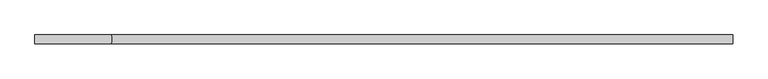
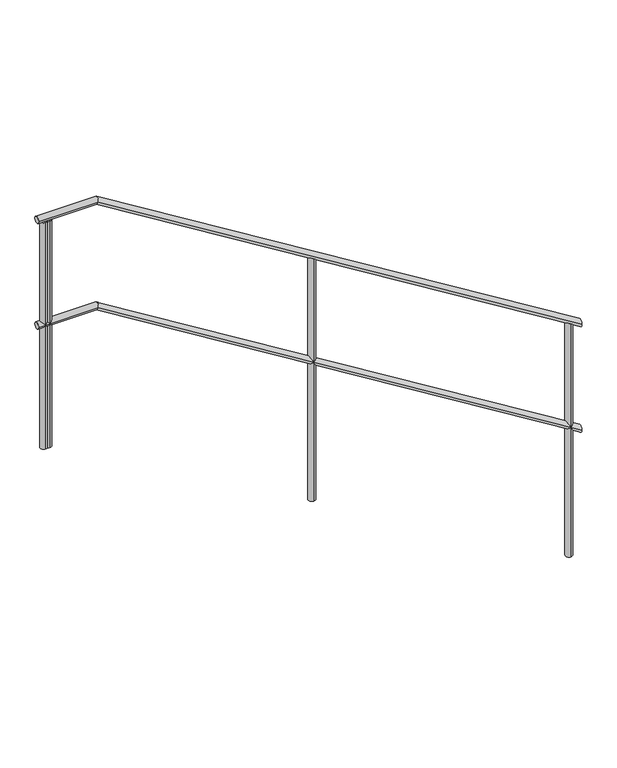
"""IFC4 building model written with IfcOpenShell, lengths in millimetres: railing geometry."""

from ifc_helpers import new_model, si_unit, point, frame, frame_2d, origin, place, context, project, spatial, circle_curve, ellipse_curve, trimmed, segment, composite_curve, outline, extrude, source, transform, mapped, element, save
from ifc_brep_helpers import plane_surface, cylinder_surface, advanced_brep


def railing_ed82b161(model_context):
    return source(origin(), model_context, "Body", "SolidModel", [
        advanced_brep(
        [(28470.0, -5867.9791411, -450.9609787), (28470.0, -5837.9791411, -450.9609787), (26305.7432145, -5867.9791411, 885.0), (26305.7432145, -5837.9791411, 885.0), (26040.0, -5867.9791411, 885.0), (26040.0, -5837.9791411, 885.0)],
        [
            (0, 1, ellipse_curve(frame((28470.0, -5852.9791411, -450.9609787), z_axis=(1.0, 0.0, 0.0), x_axis=(0.0, 0.0, -1.0)), 17.6276454, 15.0)),
            (1, 0, ellipse_curve(frame((28470.0, -5852.9791411, -450.9609787), z_axis=(1.0, 0.0, 0.0), x_axis=(0.0, 0.0, -1.0)), 17.6276454, 15.0)),
            (0, 2),
            (2, 3, ellipse_curve(frame((26305.7432145, -5852.9791411, 885.0), z_axis=(0.9620125025549406, 0.0, -0.27300539358770975), x_axis=(-0.27300539358770975, 0.0, -0.9620125025549406)), 15.5923129, 15.0)),
            (3, 1),
            (3, 2, ellipse_curve(frame((26305.7432145, -5852.9791411, 885.0), z_axis=(0.9620125025549406, 0.0, -0.27300539358770975), x_axis=(-0.27300539358770975, 0.0, -0.9620125025549406)), 15.5923129, 15.0)),
            (4, 5, circle_curve(frame((26040.0, -5852.9791411, 885.0), z_axis=(-1.0, 0.0, 0.0), x_axis=(0.0, 1.0, 0.0)), 15.0)),
            (5, 4, circle_curve(frame((26040.0, -5852.9791411, 885.0), z_axis=(-1.0, 0.0, 0.0), x_axis=(0.0, 1.0, 0.0)), 15.0)),
            (2, 4),
            (5, 3),
        ],
        [
            plane_surface(frame((28470.0, -5852.9791411, -433.3333333), z_axis=(1.0, 0.0, 0.0), x_axis=(0.0, -1.0, 0.0))),
            cylinder_surface(frame((28462.1209619, -5852.9791411, -446.097375), z_axis=(0.8509361101440394, 0.0, -0.5252692037926184), x_axis=(0.0, 1.0, 0.0)), 15.0),
            plane_surface(frame((26040.0, -5852.9791411, 900.0), z_axis=(-1.0, 0.0, 0.0), x_axis=(0.0, -1.0, 0.0))),
            cylinder_surface(frame((26310.0, -5852.9791411, 885.0), z_axis=(1.0, 0.0, 0.0), x_axis=(0.0, 1.0, 0.0)), 15.0),
        ],
        [
            (0, [[1, 2]]),
            (1, [[-1, 3, 4, 5]]),
            (1, [[-2, -5, 6, -3]]),
            (2, [[7, 8]]),
            (3, [[-4, 9, -8, 10]]),
            (3, [[-6, -10, -7, -9]]),
        ],
    ),
        advanced_brep(
        [(28470.0, -5867.9791411, 49.0390213), (28470.0, -5837.9791411, 49.0390213), (26305.7432145, -5867.9791411, 1385.0), (26305.7432145, -5837.9791411, 1385.0), (26040.0, -5867.9791411, 1385.0), (26040.0, -5837.9791411, 1385.0)],
        [
            (0, 1, ellipse_curve(frame((28470.0, -5852.9791411, 49.0390213), z_axis=(1.0, 0.0, 0.0), x_axis=(0.0, 0.0, -1.0)), 17.6276454, 15.0)),
            (1, 0, ellipse_curve(frame((28470.0, -5852.9791411, 49.0390213), z_axis=(1.0, 0.0, 0.0), x_axis=(0.0, 0.0, -1.0)), 17.6276454, 15.0)),
            (0, 2),
            (2, 3, ellipse_curve(frame((26305.7432145, -5852.9791411, 1385.0), z_axis=(0.9620125025549406, 0.0, -0.27300539358770975), x_axis=(-0.27300539358770975, 0.0, -0.9620125025549406)), 15.5923129, 15.0)),
            (3, 1),
            (3, 2, ellipse_curve(frame((26305.7432145, -5852.9791411, 1385.0), z_axis=(0.9620125025549406, 0.0, -0.27300539358770975), x_axis=(-0.27300539358770975, 0.0, -0.9620125025549406)), 15.5923129, 15.0)),
            (4, 5, circle_curve(frame((26040.0, -5852.9791411, 1385.0), z_axis=(-1.0, 0.0, 0.0), x_axis=(0.0, 1.0, 0.0)), 15.0)),
            (5, 4, circle_curve(frame((26040.0, -5852.9791411, 1385.0), z_axis=(-1.0, 0.0, 0.0), x_axis=(0.0, 1.0, 0.0)), 15.0)),
            (2, 4),
            (5, 3),
        ],
        [
            plane_surface(frame((28470.0, -5852.9791411, 66.6666667), z_axis=(1.0, 0.0, 0.0), x_axis=(0.0, -1.0, 0.0))),
            cylinder_surface(frame((28462.1209619, -5852.9791411, 53.902625), z_axis=(0.8509361101440394, 0.0, -0.5252692037926184), x_axis=(0.0, 1.0, 0.0)), 15.0),
            plane_surface(frame((26040.0, -5852.9791411, 1400.0), z_axis=(-1.0, 0.0, 0.0), x_axis=(0.0, -1.0, 0.0))),
            cylinder_surface(frame((26310.0, -5852.9791411, 1385.0), z_axis=(1.0, 0.0, 0.0), x_axis=(0.0, 1.0, 0.0)), 15.0),
        ],
        [
            (0, [[1, 2]]),
            (1, [[-1, 3, 4, 5]]),
            (1, [[-2, -5, 6, -3]]),
            (2, [[7, 8]]),
            (3, [[-4, 9, -8, 10]]),
            (3, [[-6, -10, -7, -9]]),
        ],
    ),
        extrude(outline(composite_curve([segment(trimmed(circle_curve(frame_2d((26070.0, -5852.9791411)), 15.0), [point((26070.0, -5867.9791411))], [point((26070.0, -5837.9791411))], False, "CARTESIAN"), True, "CONTINUOUS"), segment(trimmed(circle_curve(frame_2d((26070.0, -5852.9791411)), 15.0), [point((26070.0, -5837.9791411))], [point((26070.0, -5867.9791411))], False, "CARTESIAN"), True, "CONTINUOUS")], self_intersect=False)), frame((0.0, 0.0, 300.0), z_axis=(0.0, 0.0, 1.0), x_axis=(1.0, 0.0, 0.0)), (0.0, 0.0, 1.0), 1070.0),
        advanced_brep(
        [(27270.0, -5837.9791411, 777.4074074), (27270.0, -5837.9791411, -366.6666667), (27270.0, -5867.9791411, -366.6666667), (27270.0, -5867.9791411, 777.4074074)],
        [
            (0, 1),
            (1, 2, circle_curve(frame((27270.0, -5852.9791411, -366.6666667), z_axis=(0.0, 0.0, 1.0), x_axis=(0.0, -1.0, 0.0)), 15.0)),
            (2, 3),
            (3, 0, ellipse_curve(frame((27270.0, -5852.9791411, 777.4074074), z_axis=(-0.5252692037926167, 0.0, -0.8509361101440406), x_axis=(-0.8509361101440406, 0.0, 0.5252692037926162)), 17.6276454, 15.0)),
            (0, 3, ellipse_curve(frame((27270.0, -5852.9791411, 777.4074074), z_axis=(-0.5252692037926167, 0.0, -0.8509361101440406), x_axis=(-0.8509361101440406, 0.0, 0.5252692037926162)), 17.6276454, 15.0)),
            (2, 1, circle_curve(frame((27270.0, -5852.9791411, -366.6666667), z_axis=(0.0, 0.0, 1.0), x_axis=(0.0, -1.0, 0.0)), 15.0)),
        ],
        [
            cylinder_surface(frame((27270.0, -5852.9791411, -466.6666667), z_axis=(0.0, 0.0, 1.0), x_axis=(0.0, -1.0, 0.0)), 15.0),
            plane_surface(frame((27245.0, -5877.9791411, 792.8395062), z_axis=(0.5252692037926167, 0.0, 0.8509361101440406), x_axis=(0.0, 1.0, 0.0))),
            plane_surface(frame((27295.0, -5877.9791411, -366.6666667), z_axis=(0.0, 0.0, -1.0), x_axis=(0.0, 1.0, 0.0))),
        ],
        [
            (0, [[1, 2, 3, 4]]),
            (0, [[-1, 5, -3, 6]]),
            (1, [[-4, -5]]),
            (2, [[-2, -6]]),
        ],
    ),
        extrude(outline(composite_curve([segment(trimmed(circle_curve(frame_2d((26090.0, -5852.9791411)), 15.0), [point((26090.0, -5867.9791411))], [point((26090.0, -5837.9791411))], False, "CARTESIAN"), True, "CONTINUOUS"), segment(trimmed(circle_curve(frame_2d((26090.0, -5852.9791411)), 15.0), [point((26090.0, -5837.9791411))], [point((26090.0, -5867.9791411))], False, "CARTESIAN"), True, "CONTINUOUS")], self_intersect=False)), frame((0.0, 0.0, 300.0), z_axis=(0.0, 0.0, 1.0), x_axis=(1.0, 0.0, 0.0)), (0.0, 0.0, 1.0), 1070.0),
        advanced_brep(
        [(28420.0, -5837.9791411, 67.5308642), (28420.0, -5837.9791411, -1033.3333333), (28420.0, -5867.9791411, -1033.3333333), (28420.0, -5867.9791411, 67.5308642)],
        [
            (0, 1),
            (1, 2, circle_curve(frame((28420.0, -5852.9791411, -1033.3333333), z_axis=(0.0, 0.0, 1.0), x_axis=(0.0, -1.0, 0.0)), 15.0)),
            (2, 3),
            (3, 0, ellipse_curve(frame((28420.0, -5852.9791411, 67.5308642), z_axis=(-0.5252692037926167, 0.0, -0.8509361101440406), x_axis=(-0.8509361101440406, 0.0, 0.5252692037926162)), 17.6276454, 15.0)),
            (0, 3, ellipse_curve(frame((28420.0, -5852.9791411, 67.5308642), z_axis=(-0.5252692037926167, 0.0, -0.8509361101440406), x_axis=(-0.8509361101440406, 0.0, 0.5252692037926162)), 17.6276454, 15.0)),
            (2, 1, circle_curve(frame((28420.0, -5852.9791411, -1033.3333333), z_axis=(0.0, 0.0, 1.0), x_axis=(0.0, -1.0, 0.0)), 15.0)),
        ],
        [
            cylinder_surface(frame((28420.0, -5852.9791411, -1133.3333333), z_axis=(0.0, 0.0, 1.0), x_axis=(0.0, -1.0, 0.0)), 15.0),
            plane_surface(frame((28395.0, -5877.9791411, 82.962963), z_axis=(0.5252692037926167, 0.0, 0.8509361101440406), x_axis=(0.0, 1.0, 0.0))),
            plane_surface(frame((28445.0, -5877.9791411, -1033.3333333), z_axis=(0.0, 0.0, -1.0), x_axis=(0.0, 1.0, 0.0))),
        ],
        [
            (0, [[1, 2, 3, 4]]),
            (0, [[-1, 5, -3, 6]]),
            (1, [[-4, -5]]),
            (2, [[-2, -6]]),
        ],
    ),
    ])


if __name__ == "__main__":
    model = new_model("IFC4")
    model_context = context("Model", 3, world=origin())
    ifc_project = project(units=[si_unit("LENGTHUNIT", "METRE", prefix="MILLI")], contexts=[model_context])
    site = spatial("IfcSite", under=ifc_project)
    building = spatial("IfcBuilding", under=site)
    placement = place(None, origin())
    railing_shape = railing_ed82b161(model_context)
    element("IfcRailing", 1, at=placement, inside=building, context=model_context, shape_type="MappedRepresentation", body=[
        mapped(railing_shape, transform((0.0, 0.0, 0.0), x_axis=(1.0, 0.0, 0.0), y_axis=(0.0, 1.0, 0.0), z_axis=(0.0, 0.0, 1.0))),
    ])
    save(model, "model.ifc")
